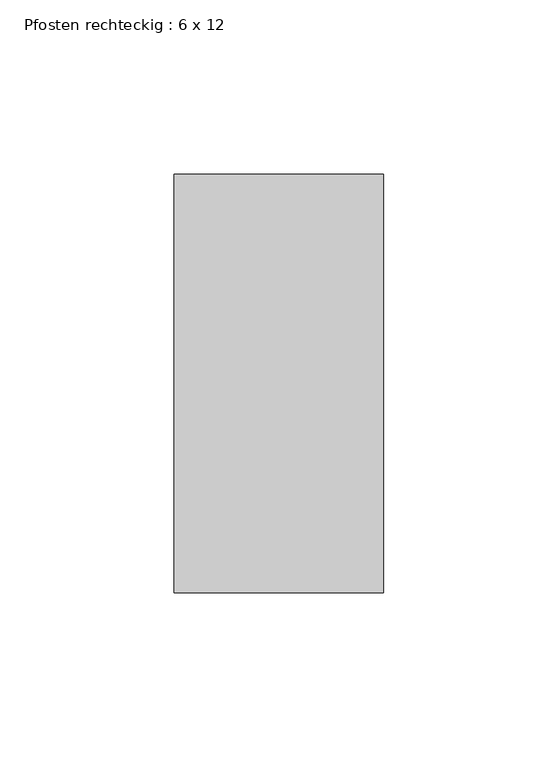
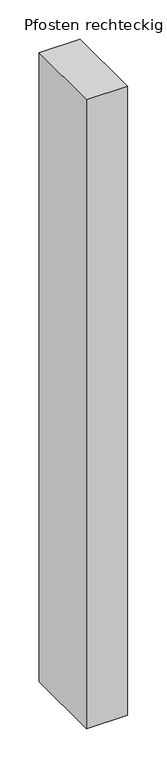
"""IFC4 building model written with IfcOpenShell, lengths in millimetres: member geometry, Pfosten rechteckig : 6 x 12."""

from ifc_helpers import new_model, si_unit, frame, origin, place, context, project, spatial, polyline, outline, extrude, source, transform, mapped, element, save


def pfosten_rechteckig_6_x_12_8927266d(model_context):
    return source(origin(), model_context, "Body", "SweptSolid", [
        extrude(outline(polyline([(30.0, 60.0), (30.0, -60.0), (-30.0, -60.0), (-30.0, 60.0), (30.0, 60.0)])), frame((0.0, 0.0, -973.2237978), z_axis=(0.0, 0.0, 1.0), x_axis=(1.0, 0.0, 0.0)), (0.0, 0.0, 1.0), 973.2237978),
    ])


if __name__ == "__main__":
    model = new_model("IFC4")
    model_context = context("Model", 3, world=origin())
    ifc_project = project(units=[si_unit("LENGTHUNIT", "METRE", prefix="MILLI")], contexts=[model_context])
    site = spatial("IfcSite", under=ifc_project)
    building = spatial("IfcBuilding", under=site)
    placement = place(None, origin())
    pfosten_rechteckig_6_x_12_shape = pfosten_rechteckig_6_x_12_8927266d(model_context)
    element("IfcMember", 1, ObjectType="Pfosten rechteckig : 6 x 12", at=placement, inside=building, context=model_context, shape_type="MappedRepresentation", body=[
        mapped(pfosten_rechteckig_6_x_12_shape, transform((0.0, 0.0, 0.0), x_axis=(1.0, 0.0, 0.0), y_axis=(0.0, 1.0, 0.0), z_axis=(0.0, 0.0, 1.0))),
    ])
    save(model, "model.ifc")

# Revit data of these elements
# Type "Pfosten rechteckig : 6 x 12"
#   built-in parameter 1007304 = 0.393701 (stored number, unit not read)
#   built-in parameter 1007301 = 0.0984252 (stored number, unit not read)
#   built-in parameter 1007300 = 0.0984252 (stored number, unit not read)
# Element 1 (IfcMember, "Pfosten rechteckig : 6 x 12")
#   Materials on its faces: "Metall - verzinkt"
# Materials
#   "Metall - verzinkt": class "Allgemeines", colour RGB 200 200 200, transparency 0, Cost = 0
